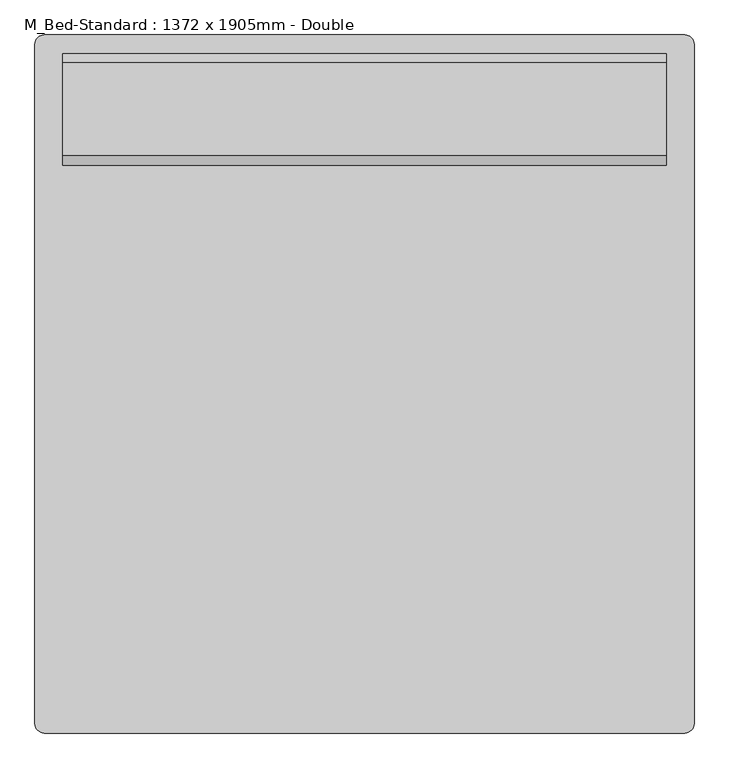
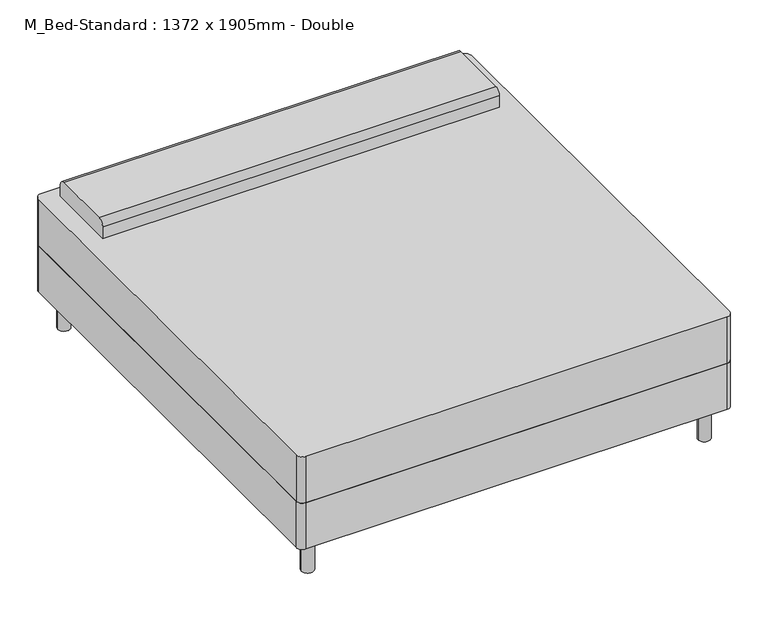
"""IFC4 building model written with IfcOpenShell, lengths in millimetres: furniture geometry, M_Bed-Standard : 1372 x 1905mm - Double."""

from ifc_helpers import new_model, si_unit, point, frame, frame_2d, origin, origin_with_axes, place, context, project, spatial, polyline, circle_curve, trimmed, segment, composite_curve, outline, extrude, source, transform, mapped, element, save


def m_bed_standard_1372_x_1905mm_double_1950cd21(model_context):
    return source(origin(), model_context, "Body", "SweptSolid", [
        extrude(outline(composite_curve([segment(polyline([(-628.5114754, -972.695082), (-628.5114754, 881.504918)]), True, "CONTINUOUS"), segment(trimmed(circle_curve(frame_2d((-603.1114754, 881.504918)), 25.4), [point((-628.5114754, 881.504918))], [point((-603.1114754, 906.904918))], False, "CARTESIAN"), True, "CONTINUOUS"), segment(polyline([(-603.1114754, 906.904918), (1146.0885246, 906.904918)]), True, "CONTINUOUS"), segment(trimmed(circle_curve(frame_2d((1146.0885246, 881.504918)), 25.4), [point((1146.0885246, 906.904918))], [point((1171.4885246, 881.504918))], False, "CARTESIAN"), True, "CONTINUOUS"), segment(polyline([(1171.4885246, 881.504918), (1171.4885246, -972.695082)]), True, "CONTINUOUS"), segment(trimmed(circle_curve(frame_2d((1146.0885246, -972.695082)), 25.4), [point((1171.4885246, -972.695082))], [point((1146.0885246, -998.095082))], False, "CARTESIAN"), True, "CONTINUOUS"), segment(polyline([(1146.0885246, -998.095082), (-603.1114754, -998.095082)]), True, "CONTINUOUS"), segment(trimmed(circle_curve(frame_2d((-603.1114754, -972.695082)), 25.4), [point((-603.1114754, -998.095082))], [point((-628.5114754, -972.695082))], False, "CARTESIAN"), True, "CONTINUOUS")], self_intersect=False)), frame((0.0, 0.0, 152.4), z_axis=(0.0, 0.0, 1.0), x_axis=(1.0, 0.0, 0.0)), (0.0, 0.0, 1.0), 203.2),
        extrude(outline(composite_curve([segment(polyline([(551.304918, 558.8), (551.304918, 609.6)]), True, "CONTINUOUS"), segment(trimmed(circle_curve(frame_2d((576.704918, 609.6)), 25.4), [point((551.304918, 609.6))], [point((576.704918, 635.0))], False, "CARTESIAN"), True, "CONTINUOUS"), segment(polyline([(576.704918, 635.0), (830.704918, 635.0)]), True, "CONTINUOUS"), segment(trimmed(circle_curve(frame_2d((830.704918, 609.6)), 25.4), [point((830.704918, 635.0))], [point((856.104918, 609.6))], False, "CARTESIAN"), True, "CONTINUOUS"), segment(polyline([(856.104918, 609.6), (856.104918, 558.8), (551.304918, 558.8)]), True, "CONTINUOUS")], self_intersect=False)), frame((-552.3114754, 0.0, 0.0), z_axis=(1.0, 0.0, 0.0), x_axis=(0.0, 1.0, 0.0)), (0.0, 0.0, 1.0), 1647.6),
        extrude(outline(composite_curve([segment(trimmed(circle_curve(frame_2d((-552.3114754, 830.704918)), 25.4), [point((-577.7114754, 830.704918))], [point((-526.9114754, 830.704918))], False, "CARTESIAN"), True, "CONTINUOUS"), segment(trimmed(circle_curve(frame_2d((-552.3114754, 830.704918)), 25.4), [point((-526.9114754, 830.704918))], [point((-577.7114754, 830.704918))], False, "CARTESIAN"), True, "CONTINUOUS")], self_intersect=False)), origin_with_axes(), (0.0, 0.0, 1.0), 152.4),
        extrude(outline(composite_curve([segment(trimmed(circle_curve(frame_2d((1095.2885246, 830.704918)), 25.4), [point((1069.8885246, 830.704918))], [point((1120.6885246, 830.704918))], False, "CARTESIAN"), True, "CONTINUOUS"), segment(trimmed(circle_curve(frame_2d((1095.2885246, 830.704918)), 25.4), [point((1120.6885246, 830.704918))], [point((1069.8885246, 830.704918))], False, "CARTESIAN"), True, "CONTINUOUS")], self_intersect=False)), origin_with_axes(), (0.0, 0.0, 1.0), 152.4),
        extrude(outline(composite_curve([segment(trimmed(circle_curve(frame_2d((1095.2885246, -921.895082)), 25.4), [point((1069.8885246, -921.895082))], [point((1120.6885246, -921.895082))], False, "CARTESIAN"), True, "CONTINUOUS"), segment(trimmed(circle_curve(frame_2d((1095.2885246, -921.895082)), 25.4), [point((1120.6885246, -921.895082))], [point((1069.8885246, -921.895082))], False, "CARTESIAN"), True, "CONTINUOUS")], self_intersect=False)), origin_with_axes(), (0.0, 0.0, 1.0), 152.4),
        extrude(outline(composite_curve([segment(trimmed(circle_curve(frame_2d((-552.3114754, -921.895082)), 25.4), [point((-577.7114754, -921.895082))], [point((-526.9114754, -921.895082))], False, "CARTESIAN"), True, "CONTINUOUS"), segment(trimmed(circle_curve(frame_2d((-552.3114754, -921.895082)), 25.4), [point((-526.9114754, -921.895082))], [point((-577.7114754, -921.895082))], False, "CARTESIAN"), True, "CONTINUOUS")], self_intersect=False)), origin_with_axes(), (0.0, 0.0, 1.0), 152.4),
        extrude(outline(composite_curve([segment(polyline([(-603.1114754, 906.904918), (1146.0885246, 906.904918)]), True, "CONTINUOUS"), segment(trimmed(circle_curve(frame_2d((1146.0885246, 881.504918)), 25.4), [point((1146.0885246, 906.904918))], [point((1171.4885246, 881.504918))], False, "CARTESIAN"), True, "CONTINUOUS"), segment(polyline([(1171.4885246, 881.504918), (1171.4885246, -972.695082)]), True, "CONTINUOUS"), segment(trimmed(circle_curve(frame_2d((1146.0885246, -972.695082)), 25.4), [point((1171.4885246, -972.695082))], [point((1146.0885246, -998.095082))], False, "CARTESIAN"), True, "CONTINUOUS"), segment(polyline([(1146.0885246, -998.095082), (-603.1114754, -998.095082)]), True, "CONTINUOUS"), segment(trimmed(circle_curve(frame_2d((-603.1114754, -972.695082)), 25.4), [point((-603.1114754, -998.095082))], [point((-628.5114754, -972.695082))], False, "CARTESIAN"), True, "CONTINUOUS"), segment(polyline([(-628.5114754, -972.695082), (-628.5114754, 881.504918)]), True, "CONTINUOUS"), segment(trimmed(circle_curve(frame_2d((-603.1114754, 881.504918)), 25.4), [point((-628.5114754, 881.504918))], [point((-603.1114754, 906.904918))], False, "CARTESIAN"), True, "CONTINUOUS")], self_intersect=False)), frame((0.0, 0.0, 355.6), z_axis=(0.0, 0.0, 1.0), x_axis=(1.0, 0.0, 0.0)), (0.0, 0.0, 1.0), 203.2),
    ])


if __name__ == "__main__":
    model = new_model("IFC4")
    model_context = context("Model", 3, world=origin())
    ifc_project = project(units=[si_unit("LENGTHUNIT", "METRE", prefix="MILLI")], contexts=[model_context])
    site = spatial("IfcSite", under=ifc_project)
    building = spatial("IfcBuilding", under=site)
    placement = place(None, origin())
    m_bed_standard_1372_x_1905mm_double_shape = m_bed_standard_1372_x_1905mm_double_1950cd21(model_context)
    element("IfcFurniture", 1, ObjectType="M_Bed-Standard : 1372 x 1905mm - Double", at=placement, inside=building, context=model_context, shape_type="MappedRepresentation", body=[
        mapped(m_bed_standard_1372_x_1905mm_double_shape, transform((0.0, 0.0, 0.0), x_axis=(1.0, 0.0, 0.0), y_axis=(0.0, 1.0, 0.0), z_axis=(0.0, 0.0, 1.0))),
    ])
    save(model, "model.ifc")

# Revit data of these elements
# Type "M_Bed-Standard : 1372 x 1905mm - Double"
#   Length = 1.905 m
#   Width = 1.8 m
#   Leg Material = Steel, Chrome Plated
#   Mattress Material = Linen, White
#   Default Elevation = 0
# Element 1 (IfcFurniture, "M_Bed-Standard : 1372 x 1905mm - Double")
#   Materials on its faces: "Linen, White", "Steel, Chrome Plated"
# Materials
#   "Steel, Chrome Plated": class "Metal", colour RGB 244 244 244, transparency 0, Description = "Chromiuim plated steel", Cost = 0
#   "Linen, White": class "Textile", colour RGB 247 247 239, transparency 0, Description = "Linen, white", Cost = 0
